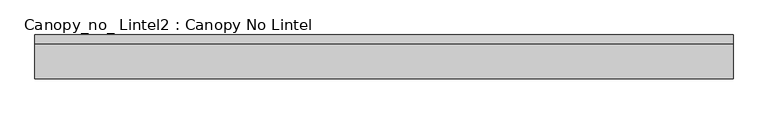
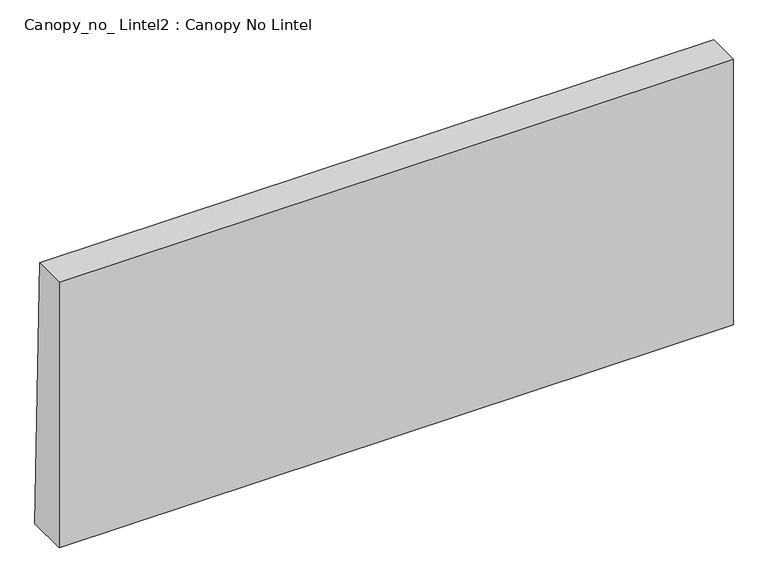
"""IFC4 building model written with IfcOpenShell, lengths in millimetres: proxy geometry, Canopy_no_ Lintel2 : Canopy No Lintel."""

from ifc_helpers import new_model, si_unit, frame, origin, place, context, project, spatial, polyline, outline, extrude, source, transform, mapped, element, save


def canopy_no_lintel2_canopy_no_lintel_c6626c79(model_context):
    return source(origin(), model_context, "Body", "SweptSolid", [
        extrude(outline(polyline([(-30.0, 1000.0), (0.0, 0.0), (-150.0, 0.0), (-150.0, 1000.0), (-30.0, 1000.0)])), frame((0.0, 0.0, 0.0), z_axis=(1.0, 0.0, 0.0), x_axis=(0.0, 1.0, 0.0)), (0.0, 0.0, 1.0), 2400.0),
    ])


if __name__ == "__main__":
    model = new_model("IFC4")
    model_context = context("Model", 3, world=origin())
    ifc_project = project(units=[si_unit("LENGTHUNIT", "METRE", prefix="MILLI")], contexts=[model_context])
    site = spatial("IfcSite", under=ifc_project)
    building = spatial("IfcBuilding", under=site)
    placement = place(None, origin())
    canopy_no_lintel2_canopy_no_lintel_shape = canopy_no_lintel2_canopy_no_lintel_c6626c79(model_context)
    element("IfcBuildingElementProxy", 1, Name="Canopy_no_ Lintel2 : Canopy No Lintel", ObjectType="Canopy_no_ Lintel2 : Canopy No Lintel", at=placement, inside=building, context=model_context, shape_type="MappedRepresentation", body=[
        mapped(canopy_no_lintel2_canopy_no_lintel_shape, transform((0.0, 0.0, 0.0), x_axis=(1.0, 0.0, 0.0), y_axis=(0.0, 1.0, 0.0), z_axis=(0.0, 0.0, 1.0))),
    ])
    save(model, "model.ifc")

# Revit data of these elements
# Type "Canopy_no_ Lintel2 : Canopy No Lintel"
#   LastUpdate = "2017-07-05 오후 5:00:05"
#   EditorName = ""
#   lintel width = 413 mm
#   lintel edge = 0 mm
#   lintel depth = 400 mm
#   d2 = 150 mm
#   d1 = 30 mm
#   W = 1000 mm
#   Length [instance default] = 2000 mm
#   Default Elevation = 1219.2 mm
#   Structure Material = none
# Element 1 (IfcBuildingElementProxy, "Canopy_no_ Lintel2 : Canopy No Lintel")
#   Length = 2400 mm
